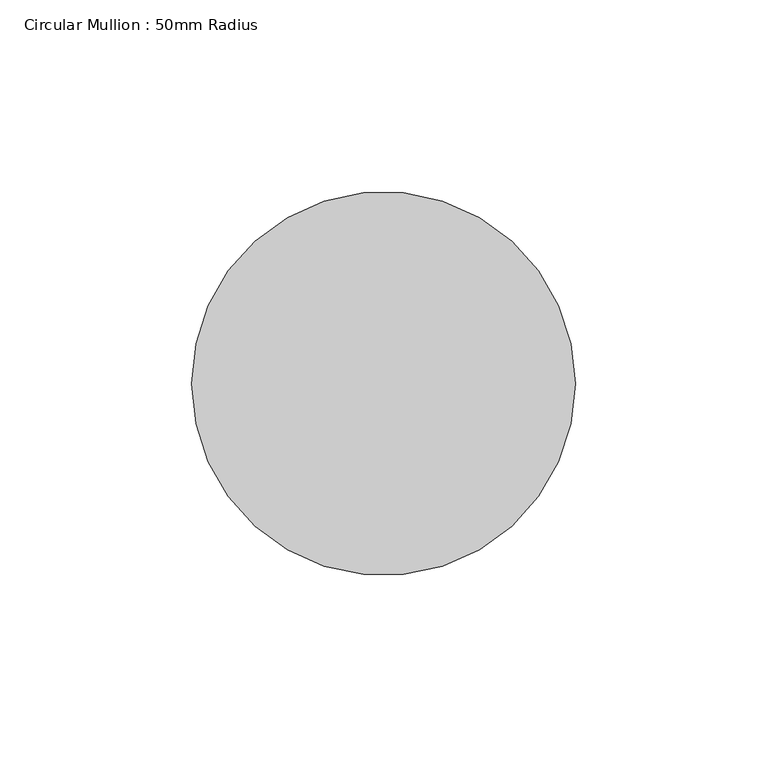
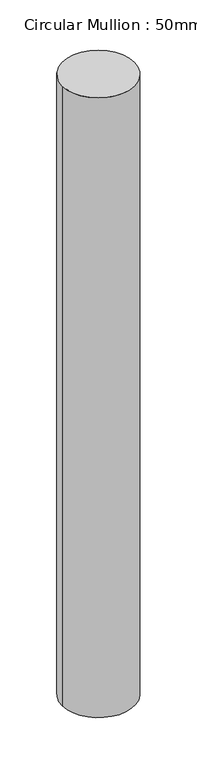
"""IFC4 building model written with IfcOpenShell, lengths in millimetres: member geometry, Circular Mullion : 50mm Radius."""

from ifc_helpers import new_model, si_unit, point, frame, origin, origin_2d, place, context, project, spatial, circle_curve, trimmed, segment, composite_curve, outline, extrude, source, transform, mapped, element, save


def circular_mullion_50mm_radius_35ab19e3(model_context):
    return source(origin(), model_context, "Body", "SweptSolid", [
        extrude(outline(composite_curve([segment(trimmed(circle_curve(origin_2d(), 50.0), [point((50.0, 0.0))], [point((-50.0, 0.0))], False, "CARTESIAN"), True, "CONTINUOUS"), segment(trimmed(circle_curve(origin_2d(), 50.0), [point((-50.0, 0.0))], [point((50.0, 0.0))], False, "CARTESIAN"), True, "CONTINUOUS")], self_intersect=False)), frame((0.0, 0.0, -909.8237099), z_axis=(0.0, 0.0, 1.0), x_axis=(1.0, 0.0, 0.0)), (0.0, 0.0, 1.0), 909.8237099),
    ])


if __name__ == "__main__":
    model = new_model("IFC4")
    model_context = context("Model", 3, world=origin())
    ifc_project = project(units=[si_unit("LENGTHUNIT", "METRE", prefix="MILLI")], contexts=[model_context])
    site = spatial("IfcSite", under=ifc_project)
    building = spatial("IfcBuilding", under=site)
    placement = place(None, origin())
    circular_mullion_50mm_radius_shape = circular_mullion_50mm_radius_35ab19e3(model_context)
    element("IfcMember", 1, ObjectType="Circular Mullion : 50mm Radius", at=placement, inside=building, context=model_context, shape_type="MappedRepresentation", body=[
        mapped(circular_mullion_50mm_radius_shape, transform((0.0, 0.0, 0.0), x_axis=(1.0, 0.0, 0.0), y_axis=(0.0, 1.0, 0.0), z_axis=(0.0, 0.0, 1.0))),
    ])
    save(model, "model.ifc")

# Revit data of these elements
# Type "Circular Mullion : 50mm Radius"
#   built-in parameter 1007350 = 0.164042 (stored number, unit not read)
# Element 1 (IfcMember, "Circular Mullion : 50mm Radius")
#   Materials on its faces: "Aluminium"
# Materials
#   "Aluminium": class "Metal", colour RGB 247 247 247, transparency 0, Description = "Aluminium 6061", Cost = 0
